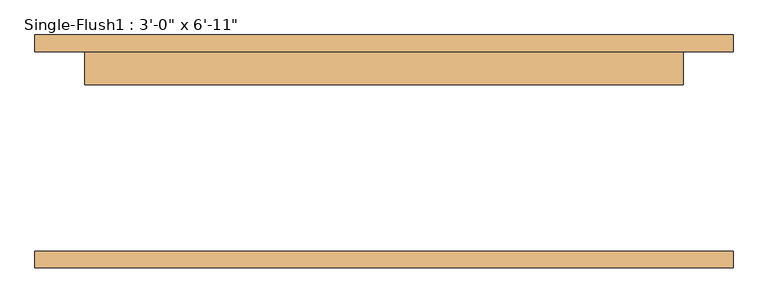
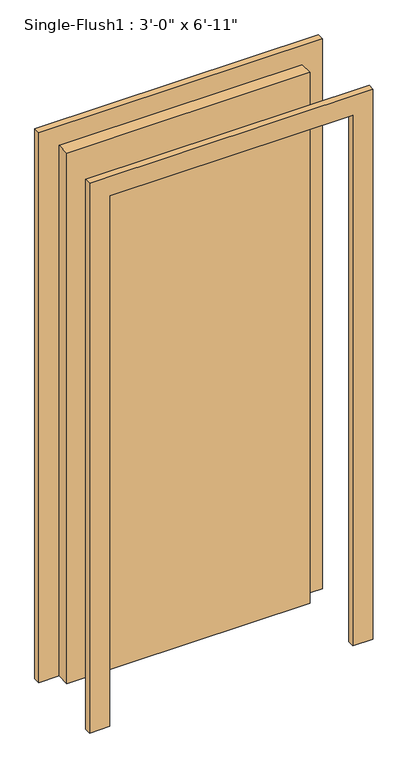
"""IFC4 building model written with IfcOpenShell, lengths in millimetres: door geometry."""

import ifcopenshell
import ifcopenshell.guid

model = None  # the IFC model being written
_history = None  # IfcOwnerHistory: only IFC2X3 demands one
_inside = {}  # id of a spatial element -> (the spatial element, [elements in it])
_under = {}  # id of a project, library or spatial element -> (it, [spatial elements below it])
_declared = {}  # id of a project -> (the project, [libraries it declares])
_typed = {}  # id of a type object -> (the type object, [elements of that type])
_made_of = {}  # id of a material, layer set ... -> (it, [elements and type objects made of it])


def new_model(schema):
    """Start an empty IFC model of exactly this schema.

    Asked for "IFC4X3", IfcOpenShell would pick the latest addendum, in which some entities
    have other attributes; the version numbers below select the first issue.
    IFC2X3 requires an IfcOwnerHistory on every rooted entity: one is made here for all.
    """
    global model, _history
    if schema == "IFC4X3":
        model = ifcopenshell.file(schema_version=(4, 3, 0, 0))
    else:
        model = ifcopenshell.file(schema=schema)
    _inside.clear()
    _under.clear()
    _declared.clear()
    _typed.clear()
    _made_of.clear()
    _history = None
    if model.schema == "IFC2X3":
        org = make("IfcOrganization", Name="unknown")
        user = make(
            "IfcPersonAndOrganization",
            ThePerson=make("IfcPerson", FamilyName="unknown"),
            TheOrganization=org,
        )
        app = make(
            "IfcApplication",
            ApplicationDeveloper=org,
            Version="unknown",
            ApplicationFullName="unknown",
            ApplicationIdentifier="unknown",
        )
        _history = make(
            "IfcOwnerHistory",
            OwningUser=user,
            OwningApplication=app,
            ChangeAction="ADDED",
            CreationDate=0,
        )
    return model


def make(cls, **values):
    """One entity of the class cls with the attributes given. An attribute that is None is left unset."""
    return model.create_entity(
        cls, **{name: value for name, value in values.items() if value is not None}
    )


def rooted(cls, **values):
    """An entity with a GlobalId (a new one), such as an element, a storey or a relation."""
    return make(cls, GlobalId=ifcopenshell.guid.new(), OwnerHistory=_history, **values)


def si_unit(unit_type, name, prefix=None):
    """IfcSIUnit, for example si_unit("LENGTHUNIT", "METRE", prefix="MILLI")."""
    return make("IfcSIUnit", UnitType=unit_type, Prefix=prefix, Name=name)


def assignment(units):
    """IfcUnitAssignment: the units of a project."""
    return None if units is None else make("IfcUnitAssignment", Units=units)


def point(xyz):
    """IfcCartesianPoint."""
    return None if xyz is None else make("IfcCartesianPoint", Coordinates=xyz)


def direction(xyz):
    """IfcDirection."""
    return None if xyz is None else make("IfcDirection", DirectionRatios=xyz)


def frame(location, z_axis=None, x_axis=None):
    """IfcAxis2Placement3D, a coordinate frame: its origin and axes. An axis left out is left unset."""
    return make(
        "IfcAxis2Placement3D",
        Location=point(location),
        Axis=direction(z_axis),
        RefDirection=direction(x_axis),
    )


def origin():
    """The frame at (0, 0, 0) with its axes left unset."""
    return frame((0.0, 0.0, 0.0))


def origin_with_axes():
    """The frame at (0, 0, 0) with the z axis (0, 0, 1) and the x axis (1, 0, 0) written out."""
    return frame((0.0, 0.0, 0.0), z_axis=(0.0, 0.0, 1.0), x_axis=(1.0, 0.0, 0.0))


def place(relative_to, where):
    """IfcLocalPlacement: puts the frame where relative to a parent placement (None: the world)."""
    return make(
        "IfcLocalPlacement", PlacementRelTo=relative_to, RelativePlacement=where
    )


def context(
    kind, dimensions, precision=None, world=None, true_north=None, identifier=None
):
    """IfcGeometricRepresentationContext, for example the 3D "Model" context."""
    return make(
        "IfcGeometricRepresentationContext",
        ContextIdentifier=identifier,
        ContextType=kind,
        CoordinateSpaceDimension=dimensions,
        Precision=precision,
        WorldCoordinateSystem=world,
        TrueNorth=true_north,
    )


def project(units=None, contexts=None):
    """IfcProject with its units and contexts."""
    return rooted(
        "IfcProject",
        Name="project",
        RepresentationContexts=contexts,
        UnitsInContext=assignment(units),
    )


def spatial(cls, under=None, at=None, **own):
    """A site, building, storey or space (cls), placed at a placement, below another one or the project."""
    s = rooted(cls, ObjectPlacement=at, **own)
    if under is not None:
        _under.setdefault(under.id(), (under, []))[1].append(s)
    return s


def polyline(points):
    """IfcPolyline through the points."""
    return make("IfcPolyline", Points=[point(p) for p in points])


def outline(outer, holes=None, kind="AREA"):
    """IfcArbitraryClosedProfileDef: a profile drawn as a closed curve; with holes, ...WithVoids."""
    if holes is None:
        return make("IfcArbitraryClosedProfileDef", ProfileType=kind, OuterCurve=outer)
    return make(
        "IfcArbitraryProfileDefWithVoids",
        ProfileType=kind,
        OuterCurve=outer,
        InnerCurves=holes,
    )


def extrude(swept, where, along, depth):
    """IfcExtrudedAreaSolid: the profile swept, set in the frame where, extruded along a direction by depth."""
    return make(
        "IfcExtrudedAreaSolid",
        SweptArea=swept,
        Position=where,
        ExtrudedDirection=direction(along),
        Depth=depth,
    )


def shape(context_of_items, identifier, shape_type, items):
    """IfcShapeRepresentation: the items that make up one representation, for example the "Body"."""
    return make(
        "IfcShapeRepresentation",
        ContextOfItems=context_of_items,
        RepresentationIdentifier=identifier,
        RepresentationType=shape_type,
        Items=items,
    )


def source(mapping_origin, context_of_items, identifier, shape_type, items):
    """IfcRepresentationMap: a shape defined once, which mapped items show again and again."""
    return make(
        "IfcRepresentationMap",
        MappingOrigin=mapping_origin,
        MappedRepresentation=shape(context_of_items, identifier, shape_type, items),
    )


def transform(
    local_origin,
    x_axis=None,
    y_axis=None,
    z_axis=None,
    scale=None,
    scale2=None,
    scale3=None,
    uniform=True,
):
    """IfcCartesianTransformationOperator3D, or its non-uniform kind. x_axis, y_axis, z_axis: its Axis1, 2, 3."""
    if uniform:
        return make(
            "IfcCartesianTransformationOperator3D",
            Axis1=direction(x_axis),
            Axis2=direction(y_axis),
            LocalOrigin=point(local_origin),
            Scale=scale,
            Axis3=direction(z_axis),
        )
    return make(
        "IfcCartesianTransformationOperator3DnonUniform",
        Axis1=direction(x_axis),
        Axis2=direction(y_axis),
        LocalOrigin=point(local_origin),
        Scale=scale,
        Axis3=direction(z_axis),
        Scale2=scale2,
        Scale3=scale3,
    )


def mapped(mapping_source, mapping_target):
    """IfcMappedItem: shows the shape of a source again, moved by a transform."""
    return make(
        "IfcMappedItem", MappingSource=mapping_source, MappingTarget=mapping_target
    )


def made_of(thing, what):
    """Note that an element or type object is made of a material, layer set ...; save() writes the relation."""
    if what is not None:
        _made_of.setdefault(what.id(), (what, []))[1].append(thing)
    return thing


def element(
    cls,
    number,
    at=None,
    inside=None,
    cuts=None,
    type_object=None,
    material=None,
    context=None,
    identifier="Body",
    shape_type=None,
    held_by="IfcProductDefinitionShape",
    body=None,
    shapes=None,
    **own,
):
    """One element of the class cls, such as IfcWall. Its Tag is "e" and its number.

    at: its placement. inside: the storey or other place that contains it. cuts: it is an
    opening in that element (IfcRelVoidsElement). A single representation is given by context,
    identifier, shape_type and body (its items); several are given by shapes. held_by: the class
    of the entity that holds the representations. save() writes the other relations.
    """
    e = rooted(cls, Tag="e%d" % number, ObjectPlacement=at, **own)
    if body is not None:
        shapes = [shape(context, identifier, shape_type, body)]
    if shapes is not None:
        e.Representation = make(held_by, Representations=shapes)
    if inside is not None:
        _inside.setdefault(inside.id(), (inside, []))[1].append(e)
    if cuts is not None:
        rooted(
            "IfcRelVoidsElement", RelatingBuildingElement=cuts, RelatedOpeningElement=e
        )
    if type_object is not None:
        _typed.setdefault(type_object.id(), (type_object, []))[1].append(e)
    return made_of(e, material)


def aggregate(whole, parts):
    """IfcRelAggregates: a whole, such as a stair, and the parts it consists of."""
    return rooted("IfcRelAggregates", RelatingObject=whole, RelatedObjects=parts)


def save(model, path):
    """Write the relations noted so far, then the file.

    IfcRelAggregates (storeys below a building ...), IfcRelContainedInSpatialStructure (elements
    in a storey), IfcRelDefinesByType, IfcRelAssociatesMaterial and IfcRelDeclares: one each for
    every whole, place, type object, material and project.
    """
    for whole, parts in _under.values():
        aggregate(whole, parts)
    for where, things in _inside.values():
        rooted(
            "IfcRelContainedInSpatialStructure",
            RelatedElements=things,
            RelatingStructure=where,
        )
    for kind, things in _typed.values():
        rooted("IfcRelDefinesByType", RelatedObjects=things, RelatingType=kind)
    for what, things in _made_of.values():
        rooted("IfcRelAssociatesMaterial", RelatedObjects=things, RelatingMaterial=what)
    for by, libraries in _declared.values():
        rooted("IfcRelDeclares", RelatingContext=by, RelatedDefinitions=libraries)
    model.write(path)


def door_a6ca3d0c(model_context):
    return source(origin(), model_context, "Body", "SweptSolid", [
        extrude(outline(polyline([(2184.4, -533.4), (0.0, -533.4), (0.0, -457.2), (2108.2, -457.2), (2108.2, 457.2), (0.0, 457.2), (0.0, 533.4), (2184.4, 533.4), (2184.4, -533.4)])), frame((0.0, 152.4, 0.0), z_axis=(0.0, 1.0, 0.0), x_axis=(0.0, 0.0, 1.0)), (0.0, 0.0, 1.0), 25.4),
        extrude(outline(polyline([(2184.4, 533.4), (2184.4, -533.4), (0.0, -533.4), (0.0, -457.2), (2108.2, -457.2), (2108.2, 457.2), (0.0, 457.2), (0.0, 533.4), (2184.4, 533.4)])), frame((0.0, -177.8, 0.0), z_axis=(0.0, 1.0, 0.0), x_axis=(0.0, 0.0, 1.0)), (0.0, 0.0, 1.0), 25.4),
        extrude(outline(polyline([(457.2, 101.6), (-457.2, 101.6), (-457.2, 152.4), (457.2, 152.4), (457.2, 101.6)])), origin_with_axes(), (0.0, 0.0, 1.0), 2108.2),
    ])


if __name__ == "__main__":
    model = new_model("IFC4")
    model_context = context("Model", 3, world=origin())
    ifc_project = project(units=[si_unit("LENGTHUNIT", "METRE", prefix="MILLI")], contexts=[model_context])
    site = spatial("IfcSite", under=ifc_project)
    building = spatial("IfcBuilding", under=site)
    placement = place(None, origin())
    door_shape = door_a6ca3d0c(model_context)
    element("IfcDoor", 1, ObjectType="Single-Flush1 : 3'-0\" x 6'-11\"", at=placement, inside=building, context=model_context, shape_type="MappedRepresentation", body=[
        mapped(door_shape, transform((0.0, 0.0, 0.0), x_axis=(1.0, 0.0, 0.0), y_axis=(0.0, 1.0, 0.0), z_axis=(0.0, 0.0, 1.0))),
    ])
    save(model, "model.ifc")

# Revit data of these elements
# Type "Single-Flush1 : 3'-0\" x 6'-11\""
#   Type Mark = "22"
#   Construction Type Id = "MDOOR"
#   Assembly Code = "C1020"
#   Analytic Construction = "Metal"
#   Thickness = 0' - 2"
#   Heat Transfer Coefficient (U) = 3.7021 W/(m²·K)
#   Height = 6' - 11"
#   Trim Projection Ext = 0' - 1"
#   Trim Projection Int = 0' - 1"
#   Trim Width = 0' - 3"
#   Width = 3' - 0"
#   Door Material = Door - Panel
#   Frame Material = Door - Frame
#   Visual Light Transmittance = 0
#   Solar Heat Gain Coefficient = 0
#   Function = (empty or 0)
#   Wall Closure = (empty or 0)
# Element 1 (IfcDoor, "Single-Flush1 : 3'-0\" x 6'-11\"")
#   Materials on its faces: "Door - Frame", "Door - Panel"
# Materials
#   "Door - Panel": class "Wood", colour RGB 210 159 95, transparency 0, Cost = 0
#   "Door - Frame": class "Miscellaneous", colour RGB 118 70 51, transparency 0, Cost = 0
